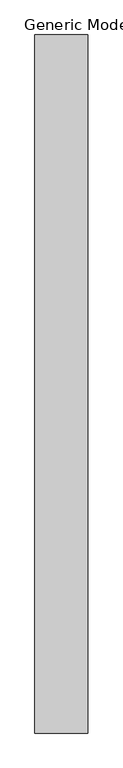
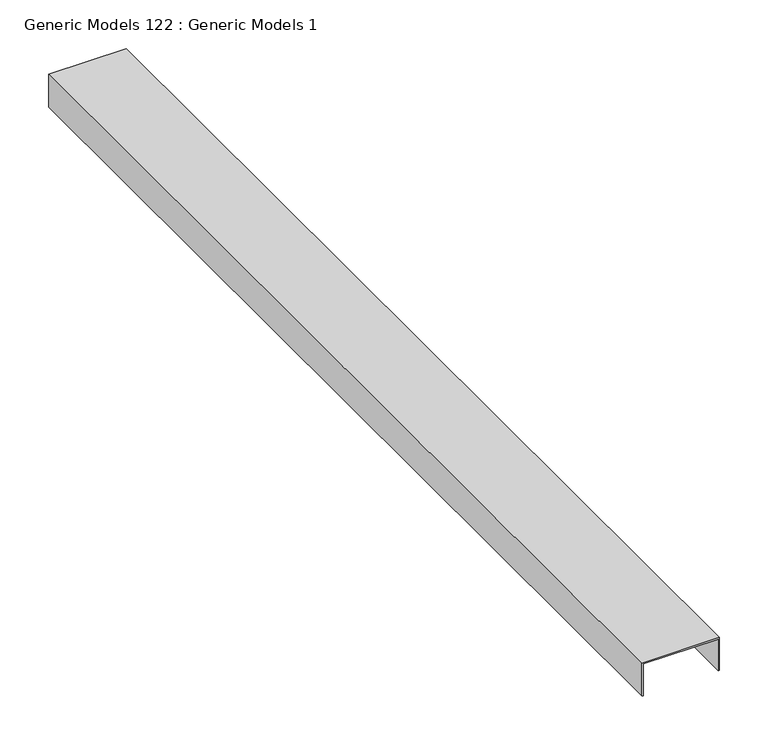
"""IFC4 building model written with IfcOpenShell, lengths in millimetres: proxy geometry, Generic Models 122 : Generic Models 1."""

from ifc_helpers import new_model, si_unit, frame, origin, place, context, project, spatial, polyline, outline, extrude, source, transform, mapped, element, save


def generic_models_122_generic_models_1_7f98dd7d(model_context):
    return source(origin(), model_context, "Body", "SweptSolid", [
        extrude(outline(polyline([(2231.473933, 46935.8735531), (2231.473933, 46843.7985531), (2190.198933, 46843.7985531), (2190.198933, 46845.3860531), (2229.886433, 46845.3860531), (2229.886433, 46934.2860531), (2190.198933, 46934.2860531), (2190.198933, 46935.8735531), (2231.473933, 46935.8735531)])), frame((0.0, 0.0, 0.0), z_axis=(0.0, 1.0, 0.0), x_axis=(0.0, 0.0, 1.0)), (0.0, 0.0, 1.0), 1219.2),
    ])


if __name__ == "__main__":
    model = new_model("IFC4")
    model_context = context("Model", 3, world=origin())
    ifc_project = project(units=[si_unit("LENGTHUNIT", "METRE", prefix="MILLI")], contexts=[model_context])
    site = spatial("IfcSite", under=ifc_project)
    building = spatial("IfcBuilding", under=site)
    placement = place(None, origin())
    generic_models_122_generic_models_1_shape = generic_models_122_generic_models_1_7f98dd7d(model_context)
    element("IfcBuildingElementProxy", 1, Name="Generic Models 122 : Generic Models 1", ObjectType="Generic Models 122 : Generic Models 1", at=placement, inside=building, context=model_context, shape_type="MappedRepresentation", body=[
        mapped(generic_models_122_generic_models_1_shape, transform((0.0, 0.0, 0.0), x_axis=(1.0, 0.0, 0.0), y_axis=(0.0, 1.0, 0.0), z_axis=(0.0, 0.0, 1.0))),
    ])
    save(model, "model.ifc")

# Revit data of these elements
# Element 1 (IfcBuildingElementProxy, "Generic Models 122 : Generic Models 1")
#   Materials on its faces: "DEEP LEG OF DEFLECTION TRACK (2\" MIN. DEFLECTION)"
# Materials
#   "DEEP LEG OF DEFLECTION TRACK (2\" MIN. DEFLECTION)": class "Unassigned", colour RGB 210 209 208, transparency 0, Keynote = "M05121300.02", Cost = 0
